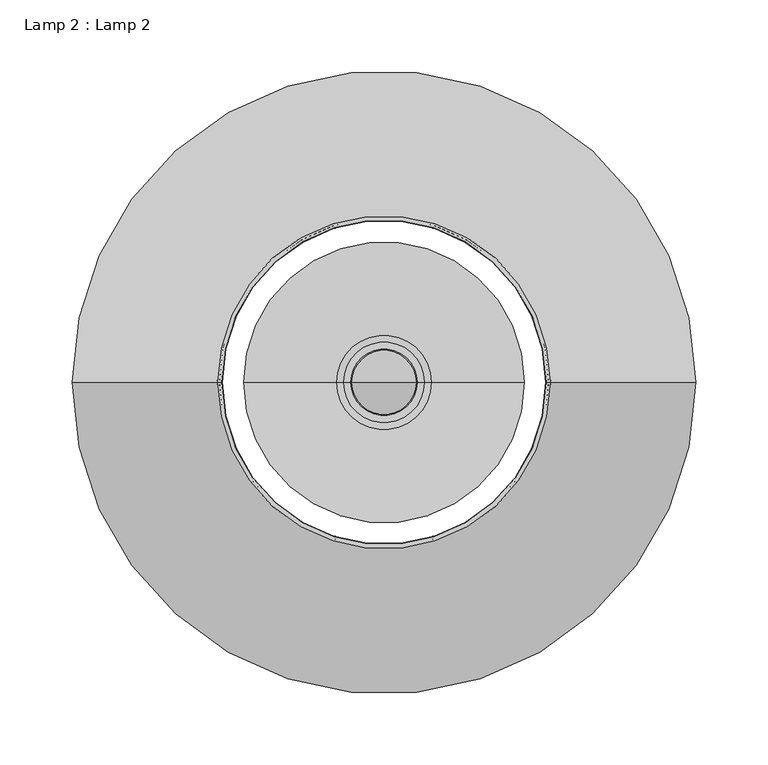
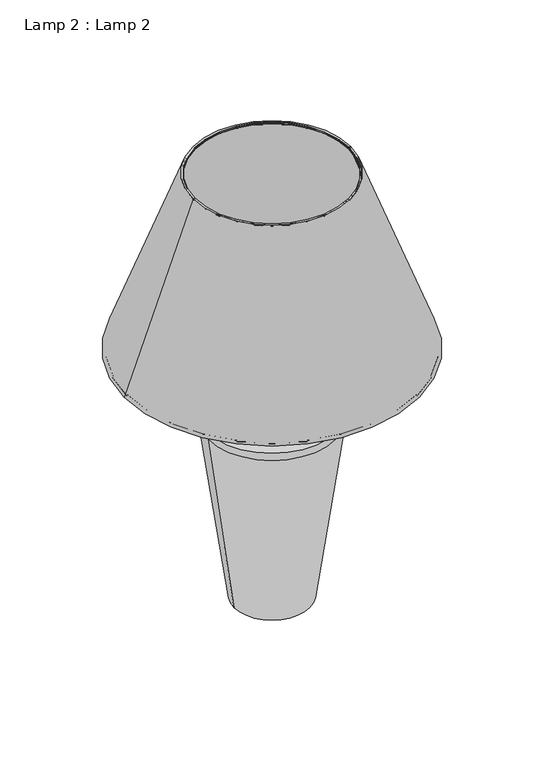
"""IFC4 building model written with IfcOpenShell, lengths in millimetres: furniture geometry, Lamp 2 : Lamp 2."""

from ifc_helpers import new_model, si_unit, point, frame, origin, place, context, project, spatial, polyline, circle_curve, ellipse_curve, trimmed, source, transform, mapped, element, save
from ifc_brep_helpers import plane_surface, cylinder_surface, revolved_surface, spline_curve, advanced_brep


def lamp_2_lamp_2_5d970a4a(model_context):
    return source(origin(), model_context, "Body", "AdvancedBrep", [
        advanced_brep(
        [(-5.625, 0.0049096, 748.6874636), (5.625, 0.0049096, 748.6874636), (5.625, 0.0049096, 736.7479044), (-5.625, 0.0049096, 736.7479044), (0.0, 0.0049096, 792.3091199), (0.0, 0.0049096, 736.7479044)],
        [
            (0, 1, circle_curve(frame((0.0, 0.0049096, 748.6874636), z_axis=(0.0, 0.0, -1.0), x_axis=(1.0, 0.0, 0.0)), 5.625)),
            (1, 2),
            (2, 3, circle_curve(frame((0.0, 0.0049096, 736.7479044), z_axis=(0.0, 0.0, 1.0), x_axis=(1.0, 0.0, 0.0)), 5.625)),
            (3, 0),
            (1, 0, circle_curve(frame((0.0, 0.0049096, 748.6874636), z_axis=(0.0, 0.0, -1.0), x_axis=(1.0, 0.0, 0.0)), 5.625)),
            (3, 2, circle_curve(frame((0.0, 0.0049096, 736.7479044), z_axis=(0.0, 0.0, 1.0), x_axis=(1.0, 0.0, 0.0)), 5.625)),
            (4, 1, circle_curve(frame((0.0, 0.0049096, 770.1356207), z_axis=(0.0, 1.0, 0.0), x_axis=(1.0, 0.0, 0.0)), 22.1734992)),
            (0, 4, circle_curve(frame((0.0, 0.0049096, 770.1356207), z_axis=(0.0, 1.0, 0.0), x_axis=(-1.0, 0.0, 0.0)), 22.1734992)),
            (2, 5),
            (5, 3),
        ],
        [
            cylinder_surface(frame((0.0, 0.0049096, 792.3091199), z_axis=(0.0, 0.0, 1.0), x_axis=(1.0, 0.0, 0.0)), 5.625),
            revolved_surface(trimmed(ellipse_curve(frame((0.0, 0.0049096, 770.1356207), z_axis=(0.0, -1.0, 0.0), x_axis=(1.0, 0.0, 0.0)), 22.1734992, 22.1734992), [point((5.625, 0.0049096, 748.6874636))], [point((0.0, 0.0049096, 792.3091199))], True, "CARTESIAN"), (0.0, 0.0049096, 792.3091199), (0.0, 0.0, 1.0)),
            plane_surface(frame((0.0, 0.0049096, 736.7479044), z_axis=(0.0, 0.0, -1.0), x_axis=(1.0, 0.0, 0.0))),
        ],
        [
            (0, [[1, 2, 3, 4]]),
            (0, [[5, -4, 6, -2]]),
            (1, [[7, -1, 8]]),
            (1, [[-8, -5, -7]]),
            (2, [[-3, 9, 10]]),
            (2, [[-6, -10, -9]]),
        ],
    ),
        advanced_brep(
        [(210.2699359, 0.0, 721.7682447), (-210.1136859, 0.0, 721.7682447), (-212.1136859, 0.0, 721.7682447), (212.2699359, 0.0, 721.7682447)],
        [
            (0, 1, circle_curve(frame((0.078125, 0.0, 721.7682447), z_axis=(0.0, 0.0, 1.0), x_axis=(-1.0, 0.0, 0.0)), 210.1918109)),
            (1, 2, circle_curve(frame((-211.1136859, 0.0, 721.7682447), z_axis=(0.0, 1.0, 0.0), x_axis=(1.0, 0.0, 0.0)), 1.0)),
            (2, 3, circle_curve(frame((0.078125, 0.0, 721.7682447), z_axis=(0.0, 0.0, -1.0), x_axis=(-1.0, 0.0, 0.0)), 212.1918109)),
            (3, 0, circle_curve(frame((211.2699359, 0.0, 721.7682447), z_axis=(0.0, 1.0, 0.0), x_axis=(-1.0, 0.0, 0.0)), 1.0)),
            (1, 0, circle_curve(frame((0.078125, 0.0, 721.7682447), z_axis=(0.0, 0.0, 1.0), x_axis=(-1.0, 0.0, 0.0)), 210.1918109)),
            (3, 2, circle_curve(frame((0.078125, 0.0, 721.7682447), z_axis=(0.0, 0.0, -1.0), x_axis=(-1.0, 0.0, 0.0)), 212.1918109)),
            (2, 1, circle_curve(frame((-211.1136859, 0.0, 721.7682447), z_axis=(0.0, 1.0, 0.0), x_axis=(1.0, 0.0, 0.0)), 1.0)),
            (0, 3, circle_curve(frame((211.2699359, 0.0, 721.7682447), z_axis=(0.0, 1.0, 0.0), x_axis=(-1.0, 0.0, 0.0)), 1.0)),
        ],
        [
            revolved_surface(trimmed(ellipse_curve(frame((-211.1136859, 0.0, 721.7682447), z_axis=(0.0, -1.0, 0.0), x_axis=(1.0, 0.0, 0.0)), 1.0, 1.0), [point((-212.1136859, 0.0, 721.7682447))], [point((-210.1136859, 0.0, 721.7682447))], True, "CARTESIAN"), (0.078125, 0.0, 710.9862512), (0.0, 0.0, -1.0)),
            revolved_surface(trimmed(ellipse_curve(frame((-211.1136859, 0.0, 721.7682447), z_axis=(0.0, -1.0, 0.0), x_axis=(1.0, 0.0, 0.0)), 1.0, 1.0), [point((-210.1136859, 0.0, 721.7682447))], [point((-212.1136859, 0.0, 721.7682447))], True, "CARTESIAN"), (0.078125, 0.0, 710.9862512), (0.0, 0.0, -1.0)),
        ],
        [
            (0, [[1, 2, 3, 4]]),
            (0, [[5, -4, 6, -2]]),
            (1, [[-3, 7, -1, 8]]),
            (1, [[-6, -8, -5, -7]]),
        ],
    ),
        advanced_brep(
        [(111.7827914, 0.0, 987.8021308), (-111.7827914, 0.0, 987.8021308), (-113.7827914, 0.0, 987.8021308), (113.7827914, 0.0, 987.8021308)],
        [
            (0, 1, circle_curve(frame((0.0, 0.0, 987.8021308), z_axis=(0.0, 0.0, 1.0), x_axis=(-1.0, 0.0, 0.0)), 111.7827914)),
            (1, 2, circle_curve(frame((-112.7827914, 0.0, 987.8021308), z_axis=(0.0, 1.0, 0.0), x_axis=(1.0, 0.0, 0.0)), 1.0)),
            (2, 3, circle_curve(frame((0.0, 0.0, 987.8021308), z_axis=(0.0, 0.0, -1.0), x_axis=(-1.0, 0.0, 0.0)), 113.7827914)),
            (3, 0, circle_curve(frame((112.7827914, 0.0, 987.8021308), z_axis=(0.0, 1.0, 0.0), x_axis=(-1.0, 0.0, 0.0)), 1.0)),
            (1, 0, circle_curve(frame((0.0, 0.0, 987.8021308), z_axis=(0.0, 0.0, 1.0), x_axis=(-1.0, 0.0, 0.0)), 111.7827914)),
            (3, 2, circle_curve(frame((0.0, 0.0, 987.8021308), z_axis=(0.0, 0.0, -1.0), x_axis=(-1.0, 0.0, 0.0)), 113.7827914)),
            (2, 1, circle_curve(frame((-112.7827914, 0.0, 987.8021308), z_axis=(0.0, 1.0, 0.0), x_axis=(1.0, 0.0, 0.0)), 1.0)),
            (0, 3, circle_curve(frame((112.7827914, 0.0, 987.8021308), z_axis=(0.0, 1.0, 0.0), x_axis=(-1.0, 0.0, 0.0)), 1.0)),
        ],
        [
            revolved_surface(trimmed(ellipse_curve(frame((-112.7827914, 0.0, 987.8021308), z_axis=(0.0, -1.0, 0.0), x_axis=(1.0, 0.0, 0.0)), 1.0, 1.0), [point((-113.7827914, 0.0, 987.8021308))], [point((-111.7827914, 0.0, 987.8021308))], True, "CARTESIAN"), (0.0, 0.0, 1009.21875), (0.0, 0.0, -1.0)),
            revolved_surface(trimmed(ellipse_curve(frame((-112.7827914, 0.0, 987.8021308), z_axis=(0.0, -1.0, 0.0), x_axis=(1.0, 0.0, 0.0)), 1.0, 1.0), [point((-111.7827914, 0.0, 987.8021308))], [point((-113.7827914, 0.0, 987.8021308))], True, "CARTESIAN"), (0.0, 0.0, 1009.21875), (0.0, 0.0, -1.0)),
        ],
        [
            (0, [[1, 2, 3, 4]]),
            (0, [[5, -4, 6, -2]]),
            (1, [[-3, 7, -1, 8]]),
            (1, [[-6, -8, -5, -7]]),
        ],
    ),
        advanced_brep(
        [(0.0, 0.0, 720.0), (-32.5, 0.0, 720.0), (32.5, 0.0, 720.0), (10.0478847, 0.0, 746.8452028), (-10.0478847, 0.0, 746.8452028), (0.0, 0.0, 746.8452028), (7.1801044, 0.0, 736.1425012), (-7.1801044, 0.0, 736.1425012), (8.4301044, 0.0, 736.1425012), (-8.4301044, 0.0, 736.1425012), (13.1200696, 0.0, 733.7368661), (-13.1200696, 0.0, 733.7368661), (13.1200696, 0.0, 730.7616675), (-13.1200696, 0.0, 730.7616675), (18.1200696, 0.0, 730.7616675), (-18.1200696, 0.0, 730.7616675), (22.8100348, 0.0, 728.3560323), (-22.8100348, 0.0, 728.3560323), (22.8100348, 0.0, 725.3808337), (-22.8100348, 0.0, 725.3808337), (27.8100348, 0.0, 725.3808337), (-27.8100348, 0.0, 725.3808337), (32.5, 0.0, 722.9751986), (-32.5, 0.0, 722.9751986)],
        [
            (0, 1),
            (1, 2, circle_curve(frame((0.0, 0.0, 720.0), z_axis=(0.0, 0.0, -1.0), x_axis=(-1.0, 0.0, 0.0)), 32.5)),
            (2, 0),
            (2, 1, circle_curve(frame((0.0, 0.0, 720.0), z_axis=(0.0, 0.0, -1.0), x_axis=(-1.0, 0.0, 0.0)), 32.5)),
            (3, 4, circle_curve(frame((0.0, 0.0, 746.8452028), z_axis=(0.0, 0.0, 1.0), x_axis=(-1.0, 0.0, 0.0)), 10.0478847)),
            (4, 5),
            (5, 3),
            (4, 3, circle_curve(frame((0.0, 0.0, 746.8452028), z_axis=(0.0, 0.0, 1.0), x_axis=(-1.0, 0.0, 0.0)), 10.0478847)),
            (6, 7, circle_curve(frame((0.0, 0.0, 736.1425012), z_axis=(0.0, 0.0, 1.0), x_axis=(-1.0, 0.0, 0.0)), 7.1801044)),
            (7, 4),
            (3, 6),
            (7, 6, circle_curve(frame((0.0, 0.0, 736.1425012), z_axis=(0.0, 0.0, 1.0), x_axis=(-1.0, 0.0, 0.0)), 7.1801044)),
            (8, 9, circle_curve(frame((0.0, 0.0, 736.1425012), z_axis=(0.0, 0.0, 1.0), x_axis=(-1.0, 0.0, 0.0)), 8.4301044)),
            (9, 7),
            (6, 8),
            (9, 8, circle_curve(frame((0.0, 0.0, 736.1425012), z_axis=(0.0, 0.0, 1.0), x_axis=(-1.0, 0.0, 0.0)), 8.4301044)),
            (10, 11, circle_curve(frame((0.0, 0.0, 733.7368661), z_axis=(0.0, 0.0, 1.0), x_axis=(-1.0, 0.0, 0.0)), 13.1200696)),
            (11, 9, circle_curve(frame((-7.7356139, 0.0, 729.0140039), z_axis=(0.0, 1.0, 0.0), x_axis=(1.0, 0.0, 0.0)), 7.1622476)),
            (8, 10, circle_curve(frame((7.7356139, 0.0, 729.0140039), z_axis=(0.0, 1.0, 0.0), x_axis=(-1.0, 0.0, 0.0)), 7.1622476)),
            (11, 10, circle_curve(frame((0.0, 0.0, 733.7368661), z_axis=(0.0, 0.0, 1.0), x_axis=(-1.0, 0.0, 0.0)), 13.1200696)),
            (12, 13, circle_curve(frame((0.0, 0.0, 730.7616675), z_axis=(0.0, 0.0, 1.0), x_axis=(-1.0, 0.0, 0.0)), 13.1200696)),
            (13, 11),
            (10, 12),
            (13, 12, circle_curve(frame((0.0, 0.0, 730.7616675), z_axis=(0.0, 0.0, 1.0), x_axis=(-1.0, 0.0, 0.0)), 13.1200696)),
            (14, 15, circle_curve(frame((0.0, 0.0, 730.7616675), z_axis=(0.0, 0.0, 1.0), x_axis=(-1.0, 0.0, 0.0)), 18.1200696)),
            (15, 13),
            (12, 14),
            (15, 14, circle_curve(frame((0.0, 0.0, 730.7616675), z_axis=(0.0, 0.0, 1.0), x_axis=(-1.0, 0.0, 0.0)), 18.1200696)),
            (16, 17, circle_curve(frame((0.0, 0.0, 728.3560323), z_axis=(0.0, 0.0, 1.0), x_axis=(-1.0, 0.0, 0.0)), 22.8100348)),
            (17, 15, circle_curve(frame((-17.4255791, 0.0, 723.6331702), z_axis=(0.0, 1.0, 0.0), x_axis=(1.0, 0.0, 0.0)), 7.1622476)),
            (14, 16, circle_curve(frame((17.4255791, 0.0, 723.6331702), z_axis=(0.0, 1.0, 0.0), x_axis=(-1.0, 0.0, 0.0)), 7.1622476)),
            (17, 16, circle_curve(frame((0.0, 0.0, 728.3560323), z_axis=(0.0, 0.0, 1.0), x_axis=(-1.0, 0.0, 0.0)), 22.8100348)),
            (18, 19, circle_curve(frame((0.0, 0.0, 725.3808337), z_axis=(0.0, 0.0, 1.0), x_axis=(-1.0, 0.0, 0.0)), 22.8100348)),
            (19, 17),
            (16, 18),
            (19, 18, circle_curve(frame((0.0, 0.0, 725.3808337), z_axis=(0.0, 0.0, 1.0), x_axis=(-1.0, 0.0, 0.0)), 22.8100348)),
            (20, 21, circle_curve(frame((0.0, 0.0, 725.3808337), z_axis=(0.0, 0.0, 1.0), x_axis=(-1.0, 0.0, 0.0)), 27.8100348)),
            (21, 19),
            (18, 20),
            (21, 20, circle_curve(frame((0.0, 0.0, 725.3808337), z_axis=(0.0, 0.0, 1.0), x_axis=(-1.0, 0.0, 0.0)), 27.8100348)),
            (22, 23, circle_curve(frame((0.0, 0.0, 722.9751986), z_axis=(0.0, 0.0, 1.0), x_axis=(-1.0, 0.0, 0.0)), 32.5)),
            (23, 21, circle_curve(frame((-27.1155443, 0.0, 718.2523365), z_axis=(0.0, 1.0, 0.0), x_axis=(1.0, 0.0, 0.0)), 7.1622476)),
            (20, 22, circle_curve(frame((27.1155443, 0.0, 718.2523365), z_axis=(0.0, 1.0, 0.0), x_axis=(-1.0, 0.0, 0.0)), 7.1622476)),
            (23, 22, circle_curve(frame((0.0, 0.0, 722.9751986), z_axis=(0.0, 0.0, 1.0), x_axis=(-1.0, 0.0, 0.0)), 32.5)),
            (1, 23),
            (22, 2),
        ],
        [
            plane_surface(frame((0.0, 0.0, 720.0), z_axis=(0.0, 0.0, -1.0), x_axis=(-1.0, 0.0, 0.0))),
            plane_surface(frame((0.0, 0.0, 746.8452028), z_axis=(0.0, 0.0, 1.0), x_axis=(-1.0, 0.0, 0.0))),
            revolved_surface(polyline([(-10.0478847, 0.0, 746.8452028), (-7.1801044, 0.0, 736.1425012)]), (0.0, 0.0, 757.9746199), (0.0, 0.0, -1.0)),
            plane_surface(frame((0.0, 0.0, 736.1425012), z_axis=(0.0, 0.0, 1.0), x_axis=(-1.0, 0.0, 0.0))),
            revolved_surface(trimmed(ellipse_curve(frame((-7.7356139, 0.0, 729.0140039), z_axis=(0.0, -1.0, 0.0), x_axis=(1.0, 0.0, 0.0)), 7.1622476, 7.1622476), [point((-8.4301044, 0.0, 736.1425012))], [point((-13.1200696, 0.0, 733.7368661))], True, "CARTESIAN"), (0.0, 0.0, 757.9746199), (0.0, 0.0, -1.0)),
            cylinder_surface(frame((0.0, 0.0, 757.9746199), z_axis=(0.0, 0.0, -1.0), x_axis=(-1.0, 0.0, 0.0)), 13.1200696),
            plane_surface(frame((0.0, 0.0, 730.7616675), z_axis=(0.0, 0.0, 1.0), x_axis=(-1.0, 0.0, 0.0))),
            revolved_surface(trimmed(ellipse_curve(frame((-17.4255791, 0.0, 723.6331702), z_axis=(0.0, -1.0, 0.0), x_axis=(1.0, 0.0, 0.0)), 7.1622476, 7.1622476), [point((-18.1200696, 0.0, 730.7616675))], [point((-22.8100348, 0.0, 728.3560323))], True, "CARTESIAN"), (0.0, 0.0, 757.9746199), (0.0, 0.0, -1.0)),
            cylinder_surface(frame((0.0, 0.0, 757.9746199), z_axis=(0.0, 0.0, -1.0), x_axis=(-1.0, 0.0, 0.0)), 22.8100348),
            plane_surface(frame((0.0, 0.0, 725.3808337), z_axis=(0.0, 0.0, 1.0), x_axis=(-1.0, 0.0, 0.0))),
            revolved_surface(trimmed(ellipse_curve(frame((-27.1155443, 0.0, 718.2523365), z_axis=(0.0, -1.0, 0.0), x_axis=(1.0, 0.0, 0.0)), 7.1622476, 7.1622476), [point((-27.8100348, 0.0, 725.3808337))], [point((-32.5, 0.0, 722.9751986))], True, "CARTESIAN"), (0.0, 0.0, 757.9746199), (0.0, 0.0, -1.0)),
            cylinder_surface(frame((0.0, 0.0, 757.9746199), z_axis=(0.0, 0.0, -1.0), x_axis=(-1.0, 0.0, 0.0)), 32.5),
        ],
        [
            (0, [[1, 2, 3]]),
            (0, [[-3, 4, -1]]),
            (1, [[5, 6, 7]]),
            (1, [[8, -7, -6]]),
            (2, [[9, 10, -5, 11]]),
            (2, [[12, -11, -8, -10]]),
            (3, [[13, 14, -9, 15]]),
            (3, [[16, -15, -12, -14]]),
            (4, [[17, 18, -13, 19]]),
            (4, [[20, -19, -16, -18]]),
            (5, [[21, 22, -17, 23]]),
            (5, [[24, -23, -20, -22]]),
            (6, [[25, 26, -21, 27]]),
            (6, [[28, -27, -24, -26]]),
            (7, [[29, 30, -25, 31]]),
            (7, [[32, -31, -28, -30]]),
            (8, [[33, 34, -29, 35]]),
            (8, [[36, -35, -32, -34]]),
            (9, [[37, 38, -33, 39]]),
            (9, [[40, -39, -36, -38]]),
            (10, [[41, 42, -37, 43]]),
            (10, [[44, -43, -40, -42]]),
            (11, [[-2, 45, -41, 46]]),
            (11, [[-4, -46, -44, -45]]),
        ],
    ),
        advanced_brep(
        [(55.0, 0.0, 340.0), (-55.0, 0.0, 340.0), (-93.2726028, 0.0, 612.3237189), (93.2726028, 0.0, 612.3237189), (0.0, 0.0, 340.0), (32.5, 0.0, 720.0), (-32.5, 0.0, 720.0), (0.0, 0.0, 720.0), (95.0446085, 0.0, 624.932195), (-95.0446085, 0.0, 624.932195)],
        [
            (0, 1, circle_curve(frame((0.0, 0.0, 340.0), z_axis=(0.0, 0.0, 1.0), x_axis=(-1.0, 0.0, 0.0)), 55.0)),
            (1, 2),
            (2, 3, circle_curve(frame((0.0, 0.0, 612.3237189), z_axis=(0.0, 0.0, -1.0), x_axis=(-1.0, 0.0, 0.0)), 93.2726028)),
            (3, 0),
            (1, 0, circle_curve(frame((0.0, 0.0, 340.0), z_axis=(0.0, 0.0, 1.0), x_axis=(-1.0, 0.0, 0.0)), 55.0)),
            (3, 2, circle_curve(frame((0.0, 0.0, 612.3237189), z_axis=(0.0, 0.0, -1.0), x_axis=(-1.0, 0.0, 0.0)), 93.2726028)),
            (4, 1),
            (0, 4),
            (5, 6, circle_curve(frame((0.0, 0.0, 720.0), z_axis=(0.0, 0.0, 1.0), x_axis=(-1.0, 0.0, 0.0)), 32.5)),
            (6, 7),
            (7, 5),
            (6, 5, circle_curve(frame((0.0, 0.0, 720.0), z_axis=(0.0, 0.0, 1.0), x_axis=(-1.0, 0.0, 0.0)), 32.5)),
            (8, 9, circle_curve(frame((0.0, 0.0, 624.932195), z_axis=(0.0, 0.0, 1.0), x_axis=(-1.0, 0.0, 0.0)), 95.0446085)),
            (9, 6, spline_curve(3, [(-95.0446085, 0.0, 624.932195), (-97.453949935, 0.0, 638.596249282), (-96.188694178, 0.0, 643.810562504), (-91.4761635, 0.0, 651.111813345), (-87.982441251, 0.0, 653.128914852), (-80.007669597, 0.0, 657.691178928), (-75.616399887, 0.0, 660.187545578), (-71.996617923, 0.0, 665.651073111), (-71.996617881, 0.0, 668.458469354), (-71.615996393, 0.0, 672.724687482), (-71.353175804, 0.0, 674.331973474), (-70.786475665, 0.0, 677.797642111), (-70.481715894, 0.0, 679.661407947), (-71.254006942, 0.0, 683.624329421), (-72.504543085, 0.0, 685.724406697), (-76.143249721, 0.0, 690.099491704), (-78.742373361, 0.0, 691.600096459), (-86.562175204, 0.0, 696.114861157), (-92.020074445, 0.0, 699.265980803), (-98.470606982, 0.0, 706.885189171), (-97.195457616, 0.0, 711.424256987), (-88.6243529, 0.0, 716.130489061), (-81.983535995, 0.0, 716.711485228), (-67.143390223, 0.0, 718.570660036), (-59.037200537, 0.0, 720.0), (-32.5, 0.0, 720.0)], [4, 2, 2, 2, 2, 2, 2, 2, 2, 2, 2, 2, 4], [0.0, 0.03985914919293754, 0.08057749635778949, 0.11834827401611286, 0.14948322781927886, 0.17098203520545735, 0.19303228957060214, 0.21777825276599289, 0.2586170795711167, 0.30356033835425955, 0.3644303221319498, 0.4188228813927918, 0.48866624030450706])),
            (5, 8, spline_curve(3, [(32.5, 0.0, 720.0), (59.037200537, 0.0, 720.0), (67.143390223, 0.0, 718.570660036), (81.983535995, 0.0, 716.711485228), (88.6243529, 0.0, 716.130489061), (97.195457616, 0.0, 711.424256987), (98.470606982, 0.0, 706.885189171), (92.020074445, 0.0, 699.265980803), (86.562175204, 0.0, 696.114861157), (78.742373361, 0.0, 691.600096459), (76.143249721, 0.0, 690.099491704), (72.504543085, 0.0, 685.724406697), (71.254006942, 0.0, 683.624329421), (70.481715894, 0.0, 679.661407947), (70.786475665, 0.0, 677.797642111), (71.353175804, 0.0, 674.331973474), (71.615996393, 0.0, 672.724687482), (71.996617881, 0.0, 668.458469354), (71.996617923, 0.0, 665.651073111), (75.616399887, 0.0, 660.187545578), (80.007669597, 0.0, 657.691178928), (87.982441251, 0.0, 653.128914852), (91.4761635, 0.0, 651.111813345), (96.188694178, 0.0, 643.810562504), (97.453949935, 0.0, 638.596249282), (95.0446085, 0.0, 624.932195)], [4, 2, 2, 2, 2, 2, 2, 2, 2, 2, 2, 2, 4], [0.0, 0.06984335891171527, 0.12423591817255722, 0.1851059019502475, 0.23004916073339038, 0.2708879875385142, 0.2956339507339049, 0.3176842050990497, 0.3391830124852282, 0.3703179662883942, 0.40808874394671757, 0.4488070911115695, 0.48866624030450706])),
            (9, 8, circle_curve(frame((0.0, 0.0, 624.932195), z_axis=(0.0, 0.0, 1.0), x_axis=(-1.0, 0.0, 0.0)), 95.0446085)),
            (2, 9),
            (8, 3),
        ],
        [
            revolved_surface(polyline([(-93.2726028, 0.0, 612.3237189), (-55.0, 0.0, 340.0)]), (0.0, 0.0, 760.0), (0.0, 0.0, -1.0)),
            plane_surface(frame((0.0, 0.0, 340.0), z_axis=(0.0, 0.0, -1.0), x_axis=(-1.0, 0.0, 0.0))),
            plane_surface(frame((0.0, 0.0, 720.0), z_axis=(0.0, 0.0, 1.0), x_axis=(-1.0, 0.0, 0.0))),
            revolved_surface(spline_curve(3, [(-32.5, 0.0, 720.0), (-59.037200537, 0.0, 720.0), (-67.143390223, 0.0, 718.570660036), (-81.983535995, 0.0, 716.711485228), (-88.6243529, 0.0, 716.130489061), (-97.195457616, 0.0, 711.424256987), (-98.470606982, 0.0, 706.885189171), (-92.020074445, 0.0, 699.265980803), (-86.562175204, 0.0, 696.114861157), (-78.742373361, 0.0, 691.600096459), (-76.143249721, 0.0, 690.099491704), (-72.504543085, 0.0, 685.724406697), (-71.254006942, 0.0, 683.624329421), (-70.481715894, 0.0, 679.661407947), (-70.786475665, 0.0, 677.797642111), (-71.353175804, 0.0, 674.331973474), (-71.615996393, 0.0, 672.724687482), (-71.996617881, 0.0, 668.458469354), (-71.996617923, 0.0, 665.651073111), (-75.616399887, 0.0, 660.187545578), (-80.007669597, 0.0, 657.691178928), (-87.982441251, 0.0, 653.128914852), (-91.4761635, 0.0, 651.111813345), (-96.188694178, 0.0, 643.810562504), (-97.453949935, 0.0, 638.596249282), (-95.0446085, 0.0, 624.932195)], [4, 2, 2, 2, 2, 2, 2, 2, 2, 2, 2, 2, 4], [0.0, 0.06984335891171527, 0.12423591817255722, 0.1851059019502475, 0.23004916073339038, 0.2708879875385142, 0.2956339507339049, 0.3176842050990497, 0.3391830124852282, 0.3703179662883942, 0.40808874394671757, 0.4488070911115695, 0.48866624030450706]), (0.0, 0.0, 760.0), (0.0, 0.0, -1.0)),
            revolved_surface(polyline([(-95.0446085, 0.0, 624.932195), (-93.2726028, 0.0, 612.3237189)]), (0.0, 0.0, 760.0), (0.0, 0.0, -1.0)),
        ],
        [
            (0, [[1, 2, 3, 4]]),
            (0, [[5, -4, 6, -2]]),
            (1, [[7, -1, 8]]),
            (1, [[-8, -5, -7]]),
            (2, [[9, 10, 11]]),
            (2, [[12, -11, -10]]),
            (3, [[13, 14, -9, 15]]),
            (3, [[16, -15, -12, -14]]),
            (4, [[-3, 17, -13, 18]]),
            (4, [[-6, -18, -16, -17]]),
        ],
    ),
        advanced_brep(
        [(-115.0, 0.0, 990.0), (115.0, 0.0, 990.0), (215.0, 0.0, 720.0), (-215.0, 0.0, 720.0), (-111.9695243, 0.0, 990.0), (111.9695243, 0.0, 990.0), (-212.7058705, 0.0, 720.7941496), (212.7058705, 0.0, 720.7941496), (113.4388971, 0.0, 988.8149779), (-113.4388971, 0.0, 988.8149779), (211.2249908, 0.0, 720.0), (-211.2249908, 0.0, 720.0), (-111.9695243, 0.0, 988.8149779), (111.9695243, 0.0, 988.8149779), (-211.2249908, 0.0, 720.7941496), (211.2249908, 0.0, 720.7941496)],
        [
            (0, 1, circle_curve(frame((0.0, 0.0, 990.0), z_axis=(0.0, 0.0, -1.0), x_axis=(1.0, 0.0, 0.0)), 115.0)),
            (1, 2),
            (2, 3, circle_curve(frame((0.0, 0.0, 720.0), z_axis=(0.0, 0.0, 1.0), x_axis=(1.0, 0.0, 0.0)), 215.0)),
            (3, 0),
            (1, 0, circle_curve(frame((0.0, 0.0, 990.0), z_axis=(0.0, 0.0, -1.0), x_axis=(1.0, 0.0, 0.0)), 115.0)),
            (3, 2, circle_curve(frame((0.0, 0.0, 720.0), z_axis=(0.0, 0.0, 1.0), x_axis=(1.0, 0.0, 0.0)), 215.0)),
            (4, 5, circle_curve(frame((0.0, 0.0, 990.0), z_axis=(0.0, 0.0, -1.0), x_axis=(1.0, 0.0, 0.0)), 111.9695243)),
            (5, 1),
            (0, 4),
            (5, 4, circle_curve(frame((0.0, 0.0, 990.0), z_axis=(0.0, 0.0, -1.0), x_axis=(1.0, 0.0, 0.0)), 111.9695243)),
            (6, 7, circle_curve(frame((0.0, 0.0, 720.7941496), z_axis=(0.0, 0.0, -1.0), x_axis=(1.0, 0.0, 0.0)), 212.7058705)),
            (7, 8),
            (8, 9, circle_curve(frame((0.0, 0.0, 988.8149779), z_axis=(0.0, 0.0, 1.0), x_axis=(1.0, 0.0, 0.0)), 113.4388971)),
            (9, 6),
            (7, 6, circle_curve(frame((0.0, 0.0, 720.7941496), z_axis=(0.0, 0.0, -1.0), x_axis=(1.0, 0.0, 0.0)), 212.7058705)),
            (9, 8, circle_curve(frame((0.0, 0.0, 988.8149779), z_axis=(0.0, 0.0, 1.0), x_axis=(1.0, 0.0, 0.0)), 113.4388971)),
            (2, 10),
            (10, 11, circle_curve(frame((0.0, 0.0, 720.0), z_axis=(0.0, 0.0, 1.0), x_axis=(1.0, 0.0, 0.0)), 211.2249908)),
            (11, 3),
            (11, 10, circle_curve(frame((0.0, 0.0, 720.0), z_axis=(0.0, 0.0, 1.0), x_axis=(1.0, 0.0, 0.0)), 211.2249908)),
            (12, 13, circle_curve(frame((0.0, 0.0, 988.8149779), z_axis=(0.0, 0.0, -1.0), x_axis=(1.0, 0.0, 0.0)), 111.9695243)),
            (13, 5),
            (4, 12),
            (13, 12, circle_curve(frame((0.0, 0.0, 988.8149779), z_axis=(0.0, 0.0, -1.0), x_axis=(1.0, 0.0, 0.0)), 111.9695243)),
            (8, 13),
            (12, 9),
            (14, 15, circle_curve(frame((0.0, 0.0, 720.7941496), z_axis=(0.0, 0.0, -1.0), x_axis=(1.0, 0.0, 0.0)), 211.2249908)),
            (15, 7),
            (6, 14),
            (15, 14, circle_curve(frame((0.0, 0.0, 720.7941496), z_axis=(0.0, 0.0, -1.0), x_axis=(1.0, 0.0, 0.0)), 211.2249908)),
            (10, 15),
            (14, 11),
        ],
        [
            revolved_surface(polyline([(215.0, 0.0, 720.0), (115.0, 0.0, 990.0)]), (0.0, 0.0, 1030.0), (0.0, 0.0, 1.0)),
            plane_surface(frame((0.0, 0.0, 990.0), z_axis=(0.0, 0.0, 1.0), x_axis=(1.0, 0.0, 0.0))),
            revolved_surface(polyline([(113.4388971, 0.0, 988.8149779), (212.7058705, 0.0, 720.7941496)]), (0.0, 0.0, 1030.0), (0.0, 0.0, 1.0)),
            plane_surface(frame((0.0, 0.0, 720.0), z_axis=(0.0, 0.0, -1.0), x_axis=(1.0, 0.0, 0.0))),
            revolved_surface(polyline([(111.9695243, 0.0, 990.0), (111.9695243, 0.0, 988.8149779)]), (0.0, 0.0, 1030.0), (0.0, 0.0, 1.0)),
            plane_surface(frame((0.0, 0.0, 988.8149779), z_axis=(0.0, 0.0, -1.0), x_axis=(1.0, 0.0, 0.0))),
            plane_surface(frame((0.0, 0.0, 720.7941496), z_axis=(0.0, 0.0, 1.0), x_axis=(1.0, 0.0, 0.0))),
            revolved_surface(polyline([(211.2249908, 0.0, 720.7941496), (211.2249908, 0.0, 720.0)]), (0.0, 0.0, 1030.0), (0.0, 0.0, 1.0)),
        ],
        [
            (0, [[1, 2, 3, 4]]),
            (0, [[5, -4, 6, -2]]),
            (1, [[7, 8, -1, 9]]),
            (1, [[10, -9, -5, -8]]),
            (2, [[11, 12, 13, 14]]),
            (2, [[15, -14, 16, -12]]),
            (3, [[-3, 17, 18, 19]]),
            (3, [[-6, -19, 20, -17]]),
            (4, [[21, 22, -7, 23]]),
            (4, [[24, -23, -10, -22]]),
            (5, [[-13, 25, -21, 26]]),
            (5, [[-16, -26, -24, -25]]),
            (6, [[27, 28, -11, 29]]),
            (6, [[30, -29, -15, -28]]),
            (7, [[-18, 31, -27, 32]]),
            (7, [[-20, -32, -30, -31]]),
        ],
    ),
    ])


if __name__ == "__main__":
    model = new_model("IFC4")
    model_context = context("Model", 3, world=origin())
    ifc_project = project(units=[si_unit("LENGTHUNIT", "METRE", prefix="MILLI")], contexts=[model_context])
    site = spatial("IfcSite", under=ifc_project)
    building = spatial("IfcBuilding", under=site)
    placement = place(None, origin())
    lamp_2_lamp_2_shape = lamp_2_lamp_2_5d970a4a(model_context)
    element("IfcFurniture", 1, ObjectType="Lamp 2 : Lamp 2", at=placement, inside=building, context=model_context, shape_type="MappedRepresentation", body=[
        mapped(lamp_2_lamp_2_shape, transform((0.0, 0.0, 0.0), x_axis=(1.0, 0.0, 0.0), y_axis=(0.0, 1.0, 0.0), z_axis=(0.0, 0.0, 1.0))),
    ])
    save(model, "model.ifc")

# Revit data of these elements
# Element 1 (IfcFurniture, "Lamp 2 : Lamp 2")
#   Materials on its faces: "Thermoplastic Resin", "Fabric Lamp Shade", "Default New Material", "Default Light Source"
# Materials
#   "Thermoplastic Resin": class "Plastic", colour RGB 255 255 125, transparency 0, Description = "Thermoplastic Resin", Cost = 0
#   "Fabric Lamp Shade": class "Generic", colour RGB 118 184 128, transparency 0.51, Cost = 0
#   "Default New Material": class "Generic", colour RGB 151 217 182, transparency 0, Description = "Porcelin", Cost = 0
#   "Default Light Source": class "System", colour RGB 255 255 0, transparency 0.75, Comments = "Rendering appearance not upgraded "
